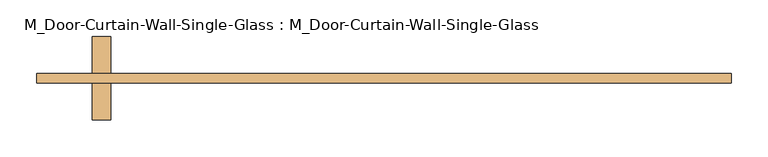
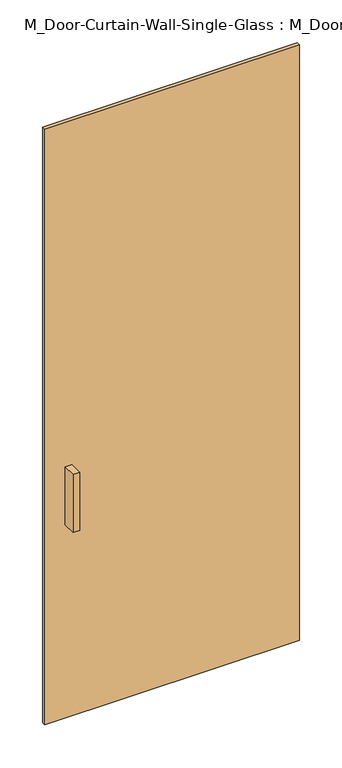
"""IFC4 building model written with IfcOpenShell, lengths in millimetres: door geometry, M_Door-Curtain-Wall-Single-Glass : M_Door-Curtain-Wall-Single-Glass."""

from ifc_helpers import new_model, si_unit, frame, origin, origin_with_axes, place, context, project, spatial, polyline, outline, extrude, source, transform, mapped, element, save


def m_door_curtain_wall_single_glass_m_door_curtain_wall_single_99f07895(model_context):
    return source(origin(), model_context, "Body", "SweptSolid", [
        extrude(outline(polyline([(475.0, -50.8), (-475.0, -50.8), (-475.0, -38.1), (475.0, -38.1), (475.0, -50.8)])), origin_with_axes(), (0.0, 0.0, 1.0), 2350.0),
        extrude(outline(polyline([(-373.4, 12.7), (-373.4, -38.1), (-398.8, -38.1), (-398.8, 12.7), (-373.4, 12.7)])), frame((0.0, 0.0, 762.0), z_axis=(0.0, 0.0, 1.0), x_axis=(1.0, 0.0, 0.0)), (0.0, 0.0, 1.0), 228.6),
        extrude(outline(polyline([(-398.8, -101.6), (-398.8, -50.8), (-373.4, -50.8), (-373.4, -101.6), (-398.8, -101.6)])), frame((0.0, 0.0, 762.0), z_axis=(0.0, 0.0, 1.0), x_axis=(1.0, 0.0, 0.0)), (0.0, 0.0, 1.0), 228.6),
    ])


if __name__ == "__main__":
    model = new_model("IFC4")
    model_context = context("Model", 3, world=origin())
    ifc_project = project(units=[si_unit("LENGTHUNIT", "METRE", prefix="MILLI")], contexts=[model_context])
    site = spatial("IfcSite", under=ifc_project)
    building = spatial("IfcBuilding", under=site)
    placement = place(None, origin())
    m_door_curtain_wall_single_glass_m_door_curtain_wall_single_shape = m_door_curtain_wall_single_glass_m_door_curtain_wall_single_99f07895(model_context)
    element("IfcDoor", 1, ObjectType="M_Door-Curtain-Wall-Single-Glass : M_Door-Curtain-Wall-Single-Glass", at=placement, inside=building, context=model_context, shape_type="MappedRepresentation", body=[
        mapped(m_door_curtain_wall_single_glass_m_door_curtain_wall_single_shape, transform((0.0, 0.0, 0.0), x_axis=(1.0, 0.0, 0.0), y_axis=(0.0, 1.0, 0.0), z_axis=(0.0, 0.0, 1.0))),
    ])
    save(model, "model.ifc")

# Revit data of these elements
# Type "M_Door-Curtain-Wall-Single-Glass : M_Door-Curtain-Wall-Single-Glass"
#   Type Mark = "50"
#   Assembly Code = "B2030100"
#   Analytic Construction = "<None>"
#   Width [instance default] = 900 mm
#   Thermal Resistance (R) = 1.7611 (m²·K)/W
#   Swing Angle [instance default] = 90.00°
#   Heat Transfer Coefficient (U) = 0.567826 W/(m²·K)
#   Offset = 50.8 mm
#   Define Thermal Properties by = 1
#   Function = 1
#   Door Handle Material = Aluminum
#   Glazing = Glass
#   Visual Light Transmittance = 0
#   Solar Heat Gain Coefficient = 0
#   Construction Type Id = ""
# Element 1 (IfcDoor, "M_Door-Curtain-Wall-Single-Glass : M_Door-Curtain-Wall-Single-Glass")
#   Width = 950 mm
#   Materials on its faces: "Aluminum", "Glass"
# Materials
#   "Aluminum": class "Metal", colour RGB 247 247 247, transparency 0, Description = "Aluminum 6061", Cost = 0
#   "Glass": class "Glass", colour RGB 0 128 192, transparency 0.9, Description = "Soda Lime Glass", Cost = 0
